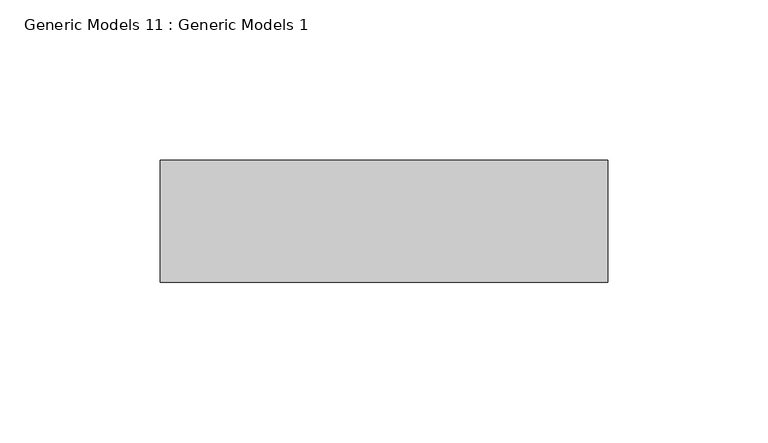
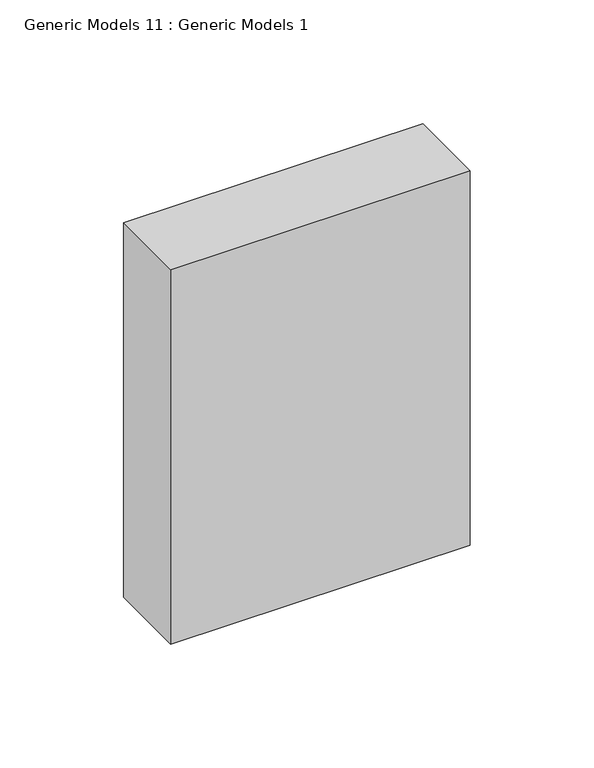
"""IFC4 building model written with IfcOpenShell, lengths in millimetres: proxy geometry, Generic Models 11 : Generic Models 1."""

from ifc_helpers import new_model, si_unit, frame, origin, place, context, project, spatial, polyline, outline, extrude, source, transform, mapped, element, save


def generic_models_11_generic_models_1_735567de(model_context):
    return source(origin(), model_context, "Body", "SweptSolid", [
        extrude(outline(polyline([(8553.2763704, 4561.4650592), (8413.5763704, 4561.4650592), (8413.5763704, 4599.5650592), (8553.2763704, 4599.5650592), (8553.2763704, 4561.4650592)])), frame((0.0, 0.0, 126821.946), z_axis=(0.0, 0.0, 1.0), x_axis=(1.0, 0.0, 0.0)), (0.0, 0.0, 1.0), 184.6825599),
    ])


if __name__ == "__main__":
    model = new_model("IFC4")
    model_context = context("Model", 3, world=origin())
    ifc_project = project(units=[si_unit("LENGTHUNIT", "METRE", prefix="MILLI")], contexts=[model_context])
    site = spatial("IfcSite", under=ifc_project)
    building = spatial("IfcBuilding", under=site)
    placement = place(None, origin())
    generic_models_11_generic_models_1_shape = generic_models_11_generic_models_1_735567de(model_context)
    element("IfcBuildingElementProxy", 1, Name="Generic Models 11 : Generic Models 1", ObjectType="Generic Models 11 : Generic Models 1", at=placement, inside=building, context=model_context, shape_type="MappedRepresentation", body=[
        mapped(generic_models_11_generic_models_1_shape, transform((0.0, 0.0, 0.0), x_axis=(1.0, 0.0, 0.0), y_axis=(0.0, 1.0, 0.0), z_axis=(0.0, 0.0, 1.0))),
    ])
    save(model, "model.ifc")

# Revit data of these elements
# Element 1 (IfcBuildingElementProxy, "Generic Models 11 : Generic Models 1")
#   Materials on its faces: "_2X BLOCKING AS REQUIRED"
# Materials
#   "_2X BLOCKING AS REQUIRED": class "Generic", colour RGB 177 130 114, transparency 0, Cost = 0
